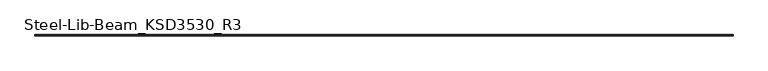
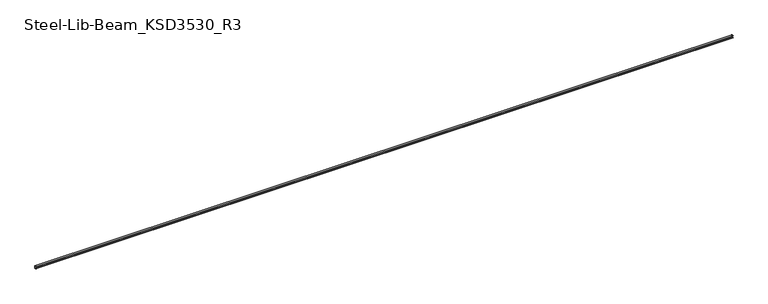
"""IFC4 building model written with IfcOpenShell, lengths in millimetres: beam geometry, Steel-Lib-Beam_KSD3530_R3 : BMS291_C-150×75x20x4.5."""

from ifc_helpers import new_model, si_unit, point, frame, frame_2d, origin, place, context, project, spatial, polyline, circle_curve, trimmed, segment, composite_curve, outline, extrude, source, transform, mapped, element, save


def steel_lib_beam_ksd3530_r3_5de18ea9(model_context):
    return source(origin(), model_context, "Body", "SweptSolid", [
        extrude(outline(composite_curve([segment(trimmed(circle_curve(frame_2d((-41.0, 66.0)), 9.0), [point((-50.0, 66.0))], [point((-41.0, 75.0))], False, "CARTESIAN"), True, "CONTINUOUS"), segment(polyline([(-41.0, 75.0), (16.0, 75.0)]), True, "CONTINUOUS"), segment(trimmed(circle_curve(frame_2d((16.0, 66.0)), 9.0), [point((16.0, 75.0))], [point((25.0, 66.0))], False, "CARTESIAN"), True, "CONTINUOUS"), segment(polyline([(25.0, 66.0), (25.0, -66.0)]), True, "CONTINUOUS"), segment(trimmed(circle_curve(frame_2d((16.0, -66.0)), 9.0), [point((25.0, -66.0))], [point((16.0, -75.0))], False, "CARTESIAN"), True, "CONTINUOUS"), segment(polyline([(16.0, -75.0), (-41.0, -75.0)]), True, "CONTINUOUS"), segment(trimmed(circle_curve(frame_2d((-41.0, -66.0)), 9.0), [point((-41.0, -75.0))], [point((-50.0, -66.0))], False, "CARTESIAN"), True, "CONTINUOUS"), segment(polyline([(-50.0, -66.0), (-50.0, -55.0), (-45.5, -55.0), (-45.5, -66.0)]), True, "CONTINUOUS"), segment(trimmed(circle_curve(frame_2d((-41.0, -66.0)), 4.5), [point((-45.5, -66.0))], [point((-41.0, -70.5))], True, "CARTESIAN"), True, "CONTINUOUS"), segment(polyline([(-41.0, -70.5), (16.0, -70.5)]), True, "CONTINUOUS"), segment(trimmed(circle_curve(frame_2d((16.0, -66.0)), 4.5), [point((16.0, -70.5))], [point((20.5, -66.0))], True, "CARTESIAN"), True, "CONTINUOUS"), segment(polyline([(20.5, -66.0), (20.5, 66.0)]), True, "CONTINUOUS"), segment(trimmed(circle_curve(frame_2d((16.0, 66.0)), 4.5), [point((20.5, 66.0))], [point((16.0, 70.5))], True, "CARTESIAN"), True, "CONTINUOUS"), segment(polyline([(16.0, 70.5), (-41.0, 70.5)]), True, "CONTINUOUS"), segment(trimmed(circle_curve(frame_2d((-41.0, 66.0)), 4.5), [point((-41.0, 70.5))], [point((-45.5, 66.0))], True, "CARTESIAN"), True, "CONTINUOUS"), segment(polyline([(-45.5, 66.0), (-45.5, 55.0), (-50.0, 55.0), (-50.0, 66.0)]), True, "CONTINUOUS")], self_intersect=False)), frame((-20547.5, 0.0, 0.0), z_axis=(1.0, 0.0, 0.0), x_axis=(0.0, 1.0, 0.0)), (0.0, 0.0, 1.0), 41095.0),
    ])


if __name__ == "__main__":
    model = new_model("IFC4")
    model_context = context("Model", 3, world=origin())
    ifc_project = project(units=[si_unit("LENGTHUNIT", "METRE", prefix="MILLI")], contexts=[model_context])
    site = spatial("IfcSite", under=ifc_project)
    building = spatial("IfcBuilding", under=site)
    placement = place(None, origin())
    steel_lib_beam_ksd3530_r3_shape = steel_lib_beam_ksd3530_r3_5de18ea9(model_context)
    element("IfcBeam", 1, ObjectType="Steel-Lib-Beam_KSD3530_R3 : BMS291_C-150×75x20x4.5", at=placement, inside=building, context=model_context, shape_type="MappedRepresentation", body=[
        mapped(steel_lib_beam_ksd3530_r3_shape, transform((0.0, 0.0, 0.0), x_axis=(1.0, 0.0, 0.0), y_axis=(0.0, 1.0, 0.0), z_axis=(0.0, 0.0, 1.0))),
    ])
    save(model, "model.ifc")

# Revit data of these elements
# Type "Steel-Lib-Beam_KSD3530_R3 : BMS291_C-150×75x20x4.5"
#   Keynote = "C-150×75x20x4.5"
#   SteelWeight = "Light"
#   x = 0.0250 m
#   t1 = 0.0090 m
#   t = 0.0045 m
#   Surface Area = 0.629834 m²/m
#   Section Area = 13.9688 cm²
#   Mass per Unit Length = 10.9655 kg/m
#   C = 0.0200 m
#   A = 0.0750 m
#   Length [instance default] = 1.5000 m
#   H = 0.1500 m
#   hec_material4 [instance default] = none
#   hec_material3 [instance default] = none
#   hec_material2 [instance default] = none
#   hec_material1 [instance default] = none
#   Structural Material [instance default] = Metal - Steel - Light Gauge
#   Assembly Code = ""
# Element 1 (IfcBeam, "Steel-Lib-Beam_KSD3530_R3 : BMS291_C-150×75x20x4.5")
#   Structural Material = none
# Materials
#   "Metal - Steel - Light Gauge": class "Metal", colour RGB 247 247 247, transparency 0
